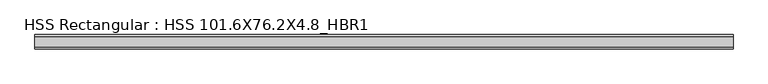
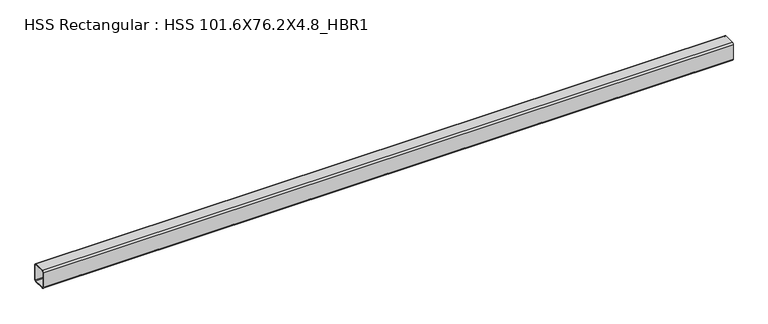
"""IFC4 building model written with IfcOpenShell, lengths in millimetres: beam geometry, HSS Rectangular : HSS 101.6X76.2X4.8_HBR1."""

from ifc_helpers import new_model, si_unit, point, frame, frame_2d, origin, place, context, project, spatial, polyline, circle_curve, trimmed, segment, composite_curve, outline, extrude, source, transform, mapped, element, save


def hss_rectangular_hss_101_6x76_2x4_8_hbr1_2c0d5523(model_context):
    return source(origin(), model_context, "Body", "SweptSolid", [
        extrude(outline(composite_curve([segment(polyline([(38.1, 41.275), (38.1, -41.275)]), True, "CONTINUOUS"), segment(trimmed(circle_curve(frame_2d((28.575, -41.275)), 9.525), [point((38.1, -41.275))], [point((28.575, -50.8))], False, "CARTESIAN"), True, "CONTINUOUS"), segment(polyline([(28.575, -50.8), (-28.575, -50.8)]), True, "CONTINUOUS"), segment(trimmed(circle_curve(frame_2d((-28.575, -41.275)), 9.525), [point((-28.575, -50.8))], [point((-38.1, -41.275))], False, "CARTESIAN"), True, "CONTINUOUS"), segment(polyline([(-38.1, -41.275), (-38.1, 41.275)]), True, "CONTINUOUS"), segment(trimmed(circle_curve(frame_2d((-28.575, 41.275)), 9.525), [point((-38.1, 41.275))], [point((-28.575, 50.8))], False, "CARTESIAN"), True, "CONTINUOUS"), segment(polyline([(-28.575, 50.8), (28.575, 50.8)]), True, "CONTINUOUS"), segment(trimmed(circle_curve(frame_2d((28.575, 41.275)), 9.525), [point((28.575, 50.8))], [point((38.1, 41.275))], False, "CARTESIAN"), True, "CONTINUOUS")], self_intersect=False), holes=[composite_curve([segment(trimmed(circle_curve(frame_2d((-28.575, 41.275)), 4.7625), [point((-28.575, 46.0375))], [point((-33.3375, 41.275))], True, "CARTESIAN"), True, "CONTINUOUS"), segment(polyline([(-33.3375, 41.275), (-33.3375, -41.275)]), True, "CONTINUOUS"), segment(trimmed(circle_curve(frame_2d((-28.575, -41.275)), 4.7625), [point((-33.3375, -41.275))], [point((-28.575, -46.0375))], True, "CARTESIAN"), True, "CONTINUOUS"), segment(polyline([(-28.575, -46.0375), (28.575, -46.0375)]), True, "CONTINUOUS"), segment(trimmed(circle_curve(frame_2d((28.575, -41.275)), 4.7625), [point((28.575, -46.0375))], [point((33.3375, -41.275))], True, "CARTESIAN"), True, "CONTINUOUS"), segment(polyline([(33.3375, -41.275), (33.3375, 41.275)]), True, "CONTINUOUS"), segment(trimmed(circle_curve(frame_2d((28.575, 41.275)), 4.7625), [point((33.3375, 41.275))], [point((28.575, 46.0375))], True, "CARTESIAN"), True, "CONTINUOUS"), segment(polyline([(28.575, 46.0375), (-28.575, 46.0375)]), True, "CONTINUOUS")], self_intersect=False)]), frame((-1860.1037503, 0.0, 0.0), z_axis=(1.0, 0.0, 0.0), x_axis=(0.0, 1.0, 0.0)), (0.0, 0.0, 1.0), 3720.925921),
    ])


if __name__ == "__main__":
    model = new_model("IFC4")
    model_context = context("Model", 3, world=origin())
    ifc_project = project(units=[si_unit("LENGTHUNIT", "METRE", prefix="MILLI")], contexts=[model_context])
    site = spatial("IfcSite", under=ifc_project)
    building = spatial("IfcBuilding", under=site)
    placement = place(None, origin())
    hss_rectangular_hss_101_6x76_2x4_8_hbr1_shape = hss_rectangular_hss_101_6x76_2x4_8_hbr1_2c0d5523(model_context)
    element("IfcBeam", 1, ObjectType="HSS Rectangular : HSS 101.6X76.2X4.8_HBR1", at=placement, inside=building, context=model_context, shape_type="MappedRepresentation", body=[
        mapped(hss_rectangular_hss_101_6x76_2x4_8_hbr1_shape, transform((0.0, 0.0, 0.0), x_axis=(1.0, 0.0, 0.0), y_axis=(0.0, 1.0, 0.0), z_axis=(0.0, 0.0, 1.0))),
    ])
    save(model, "model.ifc")

# Revit data of these elements
# Type "HSS Rectangular : HSS 101.6X76.2X4.8_HBR1"
#   Section Name Key = "HSS 4X3X3/16"
#   Assembly Code = "B10"
#   Width = 7.62 cm
#   Wall Nominal Thickness = 0.4763 cm
#   Wall Design Thickness = 0.442 cm
#   Torsional Moment of Inertia = 260.561 cm⁴
#   Torsional Modulus = 61.2876 cm³
#   Section Area = 14.4516 cm²
#   Plastic Modulus weak axis = 40.3122 cm³
#   Plastic Modulus strong axis = 49.1612 cm³
#   Perimeter = 0.881482 m²/m
#   Outer Fillet = 0.9525 cm
#   Nominal Weight = 12.1285 kgf/m
#   Moment of Inertia weak axis = 131.529 cm⁴
#   Moment of Inertia strong axis = 205.202 cm⁴
#   Inner Fillet = 0.4763 cm
#   Height = 10.16 cm
#   Elastic Modulus weak axis = 34.4128 cm³
#   Elastic Modulus strong axis = 40.476 cm³
#   Centroid Vertical = 5.08 cm
#   Centroid Horizontal = 3.81 cm
#   Length [instance default] = 1524 mm
#   Structural Material [instance default] = Steel ASTM A500, Grade B, Rectangular and Square
#   Principal Axes Angle = 0
# Element 1 (IfcBeam, "HSS Rectangular : HSS 101.6X76.2X4.8_HBR1")
#   Structural Material = Steel ASTM A992
#   Materials on its faces: "Steel ASTM A992"
# Materials
#   "Steel ASTM A500, Grade B, Rectangular and Square": class "Metal", colour RGB 199 199 199, transparency 0, Description = "Carbon steel", Cost = 0
#   "Steel ASTM A992": class "Metal", colour RGB 199 199 199, transparency 0, Description = "Structural steel 50ksi", Cost = 0
